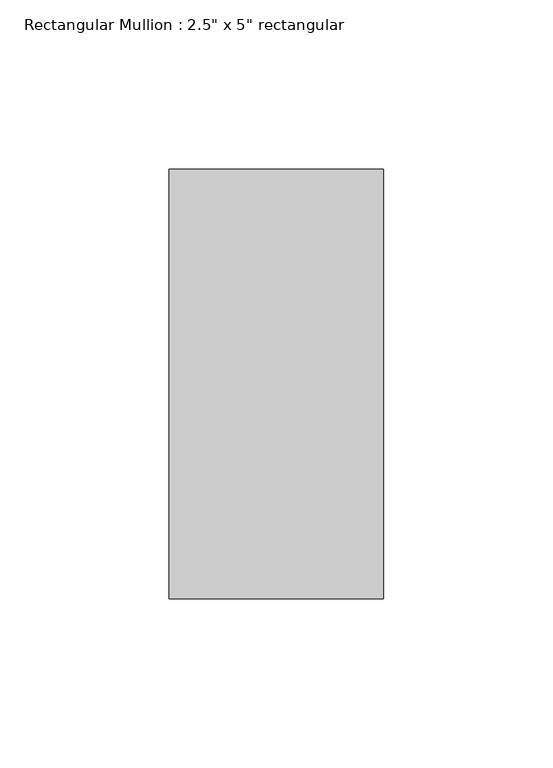
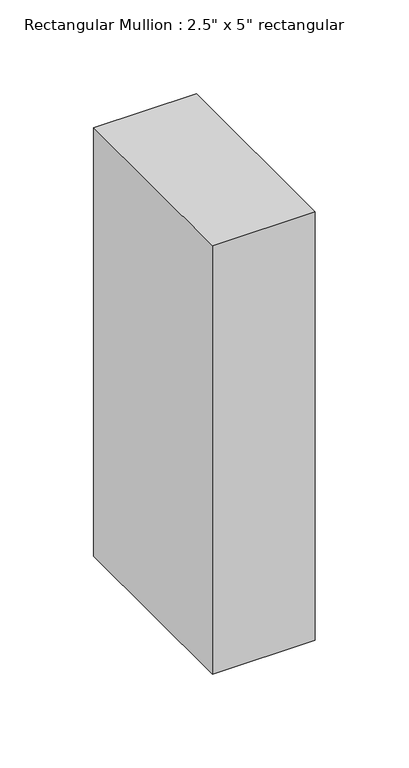
"""IFC4 building model written with IfcOpenShell, lengths in millimetres: member geometry."""

import ifcopenshell
import ifcopenshell.guid

model = None  # the IFC model being written
_history = None  # IfcOwnerHistory: only IFC2X3 demands one
_inside = {}  # id of a spatial element -> (the spatial element, [elements in it])
_under = {}  # id of a project, library or spatial element -> (it, [spatial elements below it])
_declared = {}  # id of a project -> (the project, [libraries it declares])
_typed = {}  # id of a type object -> (the type object, [elements of that type])
_made_of = {}  # id of a material, layer set ... -> (it, [elements and type objects made of it])


def new_model(schema):
    """Start an empty IFC model of exactly this schema.

    Asked for "IFC4X3", IfcOpenShell would pick the latest addendum, in which some entities
    have other attributes; the version numbers below select the first issue.
    IFC2X3 requires an IfcOwnerHistory on every rooted entity: one is made here for all.
    """
    global model, _history
    if schema == "IFC4X3":
        model = ifcopenshell.file(schema_version=(4, 3, 0, 0))
    else:
        model = ifcopenshell.file(schema=schema)
    _inside.clear()
    _under.clear()
    _declared.clear()
    _typed.clear()
    _made_of.clear()
    _history = None
    if model.schema == "IFC2X3":
        org = make("IfcOrganization", Name="unknown")
        user = make(
            "IfcPersonAndOrganization",
            ThePerson=make("IfcPerson", FamilyName="unknown"),
            TheOrganization=org,
        )
        app = make(
            "IfcApplication",
            ApplicationDeveloper=org,
            Version="unknown",
            ApplicationFullName="unknown",
            ApplicationIdentifier="unknown",
        )
        _history = make(
            "IfcOwnerHistory",
            OwningUser=user,
            OwningApplication=app,
            ChangeAction="ADDED",
            CreationDate=0,
        )
    return model


def make(cls, **values):
    """One entity of the class cls with the attributes given. An attribute that is None is left unset."""
    return model.create_entity(
        cls, **{name: value for name, value in values.items() if value is not None}
    )


def rooted(cls, **values):
    """An entity with a GlobalId (a new one), such as an element, a storey or a relation."""
    return make(cls, GlobalId=ifcopenshell.guid.new(), OwnerHistory=_history, **values)


def si_unit(unit_type, name, prefix=None):
    """IfcSIUnit, for example si_unit("LENGTHUNIT", "METRE", prefix="MILLI")."""
    return make("IfcSIUnit", UnitType=unit_type, Prefix=prefix, Name=name)


def assignment(units):
    """IfcUnitAssignment: the units of a project."""
    return None if units is None else make("IfcUnitAssignment", Units=units)


def point(xyz):
    """IfcCartesianPoint."""
    return None if xyz is None else make("IfcCartesianPoint", Coordinates=xyz)


def direction(xyz):
    """IfcDirection."""
    return None if xyz is None else make("IfcDirection", DirectionRatios=xyz)


def frame(location, z_axis=None, x_axis=None):
    """IfcAxis2Placement3D, a coordinate frame: its origin and axes. An axis left out is left unset."""
    return make(
        "IfcAxis2Placement3D",
        Location=point(location),
        Axis=direction(z_axis),
        RefDirection=direction(x_axis),
    )


def origin():
    """The frame at (0, 0, 0) with its axes left unset."""
    return frame((0.0, 0.0, 0.0))


def place(relative_to, where):
    """IfcLocalPlacement: puts the frame where relative to a parent placement (None: the world)."""
    return make(
        "IfcLocalPlacement", PlacementRelTo=relative_to, RelativePlacement=where
    )


def context(
    kind, dimensions, precision=None, world=None, true_north=None, identifier=None
):
    """IfcGeometricRepresentationContext, for example the 3D "Model" context."""
    return make(
        "IfcGeometricRepresentationContext",
        ContextIdentifier=identifier,
        ContextType=kind,
        CoordinateSpaceDimension=dimensions,
        Precision=precision,
        WorldCoordinateSystem=world,
        TrueNorth=true_north,
    )


def project(units=None, contexts=None):
    """IfcProject with its units and contexts."""
    return rooted(
        "IfcProject",
        Name="project",
        RepresentationContexts=contexts,
        UnitsInContext=assignment(units),
    )


def spatial(cls, under=None, at=None, **own):
    """A site, building, storey or space (cls), placed at a placement, below another one or the project."""
    s = rooted(cls, ObjectPlacement=at, **own)
    if under is not None:
        _under.setdefault(under.id(), (under, []))[1].append(s)
    return s


def polyline(points):
    """IfcPolyline through the points."""
    return make("IfcPolyline", Points=[point(p) for p in points])


def outline(outer, holes=None, kind="AREA"):
    """IfcArbitraryClosedProfileDef: a profile drawn as a closed curve; with holes, ...WithVoids."""
    if holes is None:
        return make("IfcArbitraryClosedProfileDef", ProfileType=kind, OuterCurve=outer)
    return make(
        "IfcArbitraryProfileDefWithVoids",
        ProfileType=kind,
        OuterCurve=outer,
        InnerCurves=holes,
    )


def extrude(swept, where, along, depth):
    """IfcExtrudedAreaSolid: the profile swept, set in the frame where, extruded along a direction by depth."""
    return make(
        "IfcExtrudedAreaSolid",
        SweptArea=swept,
        Position=where,
        ExtrudedDirection=direction(along),
        Depth=depth,
    )


def shape(context_of_items, identifier, shape_type, items):
    """IfcShapeRepresentation: the items that make up one representation, for example the "Body"."""
    return make(
        "IfcShapeRepresentation",
        ContextOfItems=context_of_items,
        RepresentationIdentifier=identifier,
        RepresentationType=shape_type,
        Items=items,
    )


def source(mapping_origin, context_of_items, identifier, shape_type, items):
    """IfcRepresentationMap: a shape defined once, which mapped items show again and again."""
    return make(
        "IfcRepresentationMap",
        MappingOrigin=mapping_origin,
        MappedRepresentation=shape(context_of_items, identifier, shape_type, items),
    )


def transform(
    local_origin,
    x_axis=None,
    y_axis=None,
    z_axis=None,
    scale=None,
    scale2=None,
    scale3=None,
    uniform=True,
):
    """IfcCartesianTransformationOperator3D, or its non-uniform kind. x_axis, y_axis, z_axis: its Axis1, 2, 3."""
    if uniform:
        return make(
            "IfcCartesianTransformationOperator3D",
            Axis1=direction(x_axis),
            Axis2=direction(y_axis),
            LocalOrigin=point(local_origin),
            Scale=scale,
            Axis3=direction(z_axis),
        )
    return make(
        "IfcCartesianTransformationOperator3DnonUniform",
        Axis1=direction(x_axis),
        Axis2=direction(y_axis),
        LocalOrigin=point(local_origin),
        Scale=scale,
        Axis3=direction(z_axis),
        Scale2=scale2,
        Scale3=scale3,
    )


def mapped(mapping_source, mapping_target):
    """IfcMappedItem: shows the shape of a source again, moved by a transform."""
    return make(
        "IfcMappedItem", MappingSource=mapping_source, MappingTarget=mapping_target
    )


def made_of(thing, what):
    """Note that an element or type object is made of a material, layer set ...; save() writes the relation."""
    if what is not None:
        _made_of.setdefault(what.id(), (what, []))[1].append(thing)
    return thing


def element(
    cls,
    number,
    at=None,
    inside=None,
    cuts=None,
    type_object=None,
    material=None,
    context=None,
    identifier="Body",
    shape_type=None,
    held_by="IfcProductDefinitionShape",
    body=None,
    shapes=None,
    **own,
):
    """One element of the class cls, such as IfcWall. Its Tag is "e" and its number.

    at: its placement. inside: the storey or other place that contains it. cuts: it is an
    opening in that element (IfcRelVoidsElement). A single representation is given by context,
    identifier, shape_type and body (its items); several are given by shapes. held_by: the class
    of the entity that holds the representations. save() writes the other relations.
    """
    e = rooted(cls, Tag="e%d" % number, ObjectPlacement=at, **own)
    if body is not None:
        shapes = [shape(context, identifier, shape_type, body)]
    if shapes is not None:
        e.Representation = make(held_by, Representations=shapes)
    if inside is not None:
        _inside.setdefault(inside.id(), (inside, []))[1].append(e)
    if cuts is not None:
        rooted(
            "IfcRelVoidsElement", RelatingBuildingElement=cuts, RelatedOpeningElement=e
        )
    if type_object is not None:
        _typed.setdefault(type_object.id(), (type_object, []))[1].append(e)
    return made_of(e, material)


def aggregate(whole, parts):
    """IfcRelAggregates: a whole, such as a stair, and the parts it consists of."""
    return rooted("IfcRelAggregates", RelatingObject=whole, RelatedObjects=parts)


def save(model, path):
    """Write the relations noted so far, then the file.

    IfcRelAggregates (storeys below a building ...), IfcRelContainedInSpatialStructure (elements
    in a storey), IfcRelDefinesByType, IfcRelAssociatesMaterial and IfcRelDeclares: one each for
    every whole, place, type object, material and project.
    """
    for whole, parts in _under.values():
        aggregate(whole, parts)
    for where, things in _inside.values():
        rooted(
            "IfcRelContainedInSpatialStructure",
            RelatedElements=things,
            RelatingStructure=where,
        )
    for kind, things in _typed.values():
        rooted("IfcRelDefinesByType", RelatedObjects=things, RelatingType=kind)
    for what, things in _made_of.values():
        rooted("IfcRelAssociatesMaterial", RelatedObjects=things, RelatingMaterial=what)
    for by, libraries in _declared.values():
        rooted("IfcRelDeclares", RelatingContext=by, RelatedDefinitions=libraries)
    model.write(path)


def member_d3323a85(model_context):
    return source(origin(), model_context, "Body", "SweptSolid", [
        extrude(outline(polyline([(0.0, 63.5), (0.0, -63.5), (-63.5, -63.5), (-63.5, 63.5), (0.0, 63.5)])), frame((0.0, 0.0, -279.4), z_axis=(0.0, 0.0, 1.0), x_axis=(1.0, 0.0, 0.0)), (0.0, 0.0, 1.0), 279.4),
    ])


if __name__ == "__main__":
    model = new_model("IFC4")
    model_context = context("Model", 3, world=origin())
    ifc_project = project(units=[si_unit("LENGTHUNIT", "METRE", prefix="MILLI")], contexts=[model_context])
    site = spatial("IfcSite", under=ifc_project)
    building = spatial("IfcBuilding", under=site)
    placement = place(None, origin())
    member_shape = member_d3323a85(model_context)
    element("IfcMember", 1, ObjectType="Rectangular Mullion : 2.5\" x 5\" rectangular", at=placement, inside=building, context=model_context, shape_type="MappedRepresentation", body=[
        mapped(member_shape, transform((0.0, 0.0, 0.0), x_axis=(1.0, 0.0, 0.0), y_axis=(0.0, 1.0, 0.0), z_axis=(0.0, 0.0, 1.0))),
    ])
    save(model, "model.ifc")

# Revit data of these elements
# Type "Rectangular Mullion : 2.5\" x 5\" rectangular"
#   built-in parameter 1007304 = 0.416667 (stored number, unit not read)
#   built-in parameter 1007301 = 0.104167 (stored number, unit not read)
#   built-in parameter 1007300 = 0.104167 (stored number, unit not read)
# Element 1 (IfcMember, "Rectangular Mullion : 2.5\" x 5\" rectangular")
#   Materials on its faces: "Metal - Aluminum"
# Materials
#   "Metal - Aluminum": class "Metal", colour RGB 140 140 140, transparency 0
